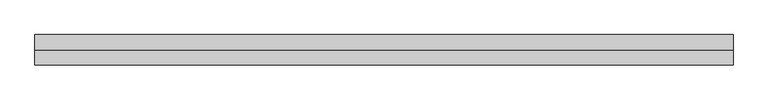
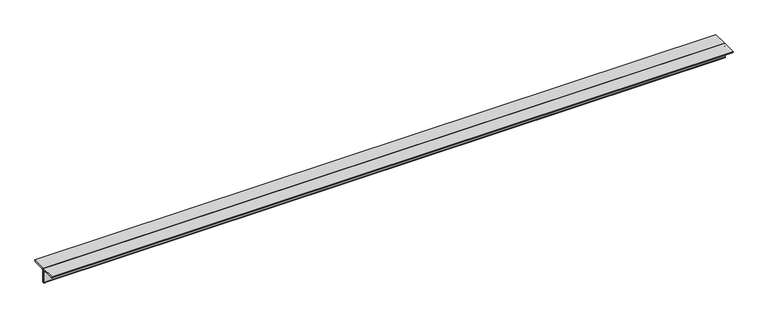
"""IFC4 building model written with IfcOpenShell, lengths in millimetres: member geometry, 0123_Steel Framing_2Ls-KSD3502 : H_SB_AR_S03_2Ls-130x130x12_HBR1."""

from ifc_helpers import new_model, si_unit, point, frame, frame_2d, origin, place, context, project, spatial, polyline, circle_curve, trimmed, segment, composite_curve, outline, extrude, source, transform, mapped, element, save


def member_93b6b39c(model_context):
    return source(origin(), model_context, "Body", "SweptSolid", [
        extrude(outline(composite_curve([segment(polyline([(0.0, 36.4), (130.0, 36.4)]), True, "CONTINUOUS"), segment(trimmed(circle_curve(frame_2d((118.0, 36.4)), 12.0), [point((130.0, 36.4))], [point((118.0, 24.4))], False, "CARTESIAN"), True, "CONTINUOUS"), segment(polyline([(118.0, 24.4), (24.0, 24.4)]), True, "CONTINUOUS"), segment(trimmed(circle_curve(frame_2d((24.0, 12.4)), 12.0), [point((24.0, 24.4))], [point((12.0, 12.4))], True, "CARTESIAN"), True, "CONTINUOUS"), segment(polyline([(12.0, 12.4), (12.0, -81.6)]), True, "CONTINUOUS"), segment(trimmed(circle_curve(frame_2d((0.0, -81.6)), 12.0), [point((12.0, -81.6))], [point((0.0, -93.6))], False, "CARTESIAN"), True, "CONTINUOUS"), segment(polyline([(0.0, -93.6), (0.0, 36.4)]), True, "CONTINUOUS")], self_intersect=False)), frame((-2923.1123523, 0.0, 0.0), z_axis=(1.0, 0.0, 0.0), x_axis=(0.0, 1.0, 0.0)), (0.0, 0.0, 1.0), 5953.2348533),
        extrude(outline(composite_curve([segment(polyline([(0.0, 36.4), (0.0, -93.6)]), True, "CONTINUOUS"), segment(trimmed(circle_curve(frame_2d((0.0, -81.6)), 12.0), [point((0.0, -93.6))], [point((-12.0, -81.6))], False, "CARTESIAN"), True, "CONTINUOUS"), segment(polyline([(-12.0, -81.6), (-12.0, 12.4)]), True, "CONTINUOUS"), segment(trimmed(circle_curve(frame_2d((-24.0, 12.4)), 12.0), [point((-12.0, 12.4))], [point((-24.0, 24.4))], True, "CARTESIAN"), True, "CONTINUOUS"), segment(polyline([(-24.0, 24.4), (-118.0, 24.4)]), True, "CONTINUOUS"), segment(trimmed(circle_curve(frame_2d((-118.0, 36.4)), 12.0), [point((-118.0, 24.4))], [point((-130.0, 36.4))], False, "CARTESIAN"), True, "CONTINUOUS"), segment(polyline([(-130.0, 36.4), (0.0, 36.4)]), True, "CONTINUOUS")], self_intersect=False)), frame((-2923.1123523, 0.0, 0.0), z_axis=(1.0, 0.0, 0.0), x_axis=(0.0, 1.0, 0.0)), (0.0, 0.0, 1.0), 5953.2348533),
    ])


if __name__ == "__main__":
    model = new_model("IFC4")
    model_context = context("Model", 3, world=origin())
    ifc_project = project(units=[si_unit("LENGTHUNIT", "METRE", prefix="MILLI")], contexts=[model_context])
    site = spatial("IfcSite", under=ifc_project)
    building = spatial("IfcBuilding", under=site)
    placement = place(None, origin())
    member_shape = member_93b6b39c(model_context)
    element("IfcMember", 1, ObjectType="0123_Steel Framing_2Ls-KSD3502 : H_SB_AR_S03_2Ls-130x130x12_HBR1", at=placement, inside=building, context=model_context, shape_type="MappedRepresentation", body=[
        mapped(member_shape, transform((0.0, 0.0, 0.0), x_axis=(1.0, 0.0, 0.0), y_axis=(0.0, 1.0, 0.0), z_axis=(0.0, 0.0, 1.0))),
    ])
    save(model, "model.ifc")

# Revit data of these elements
# Type "0123_Steel Framing_2Ls-KSD3502 : H_SB_AR_S03_2Ls-130x130x12_HBR1"
#   Type Mark = "HBR1"
#   Assembly Code = "B10"
#   Legs = "SLBB"
#   W = 8.97
#   Perimeter = 1.04 m²/m
#   Nominal Weight = 46.80 kgf/m
#   Length [instance default] = 1000 mm
#   Space = 0 mm
#   b = 130 mm
#   d = 130 mm
#   t = 12 mm
#   y = 36.4 mm
#   A = 0.005952 m²
#   Structural Material [instance default] = Steel ASTM A36
# Element 1 (IfcMember, "0123_Steel Framing_2Ls-KSD3502 : H_SB_AR_S03_2Ls-130x130x12_HBR1")
#   Materials on its faces: "Steel ASTM A36"
# Materials
#   "Steel ASTM A36": class "Metal", colour RGB 199 199 199, transparency 0, Description = "Structural steel, ASTM A36 Grade B, mill finish", Cost = 0
